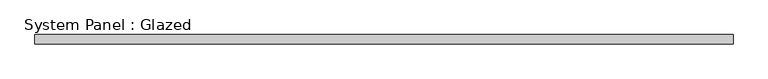
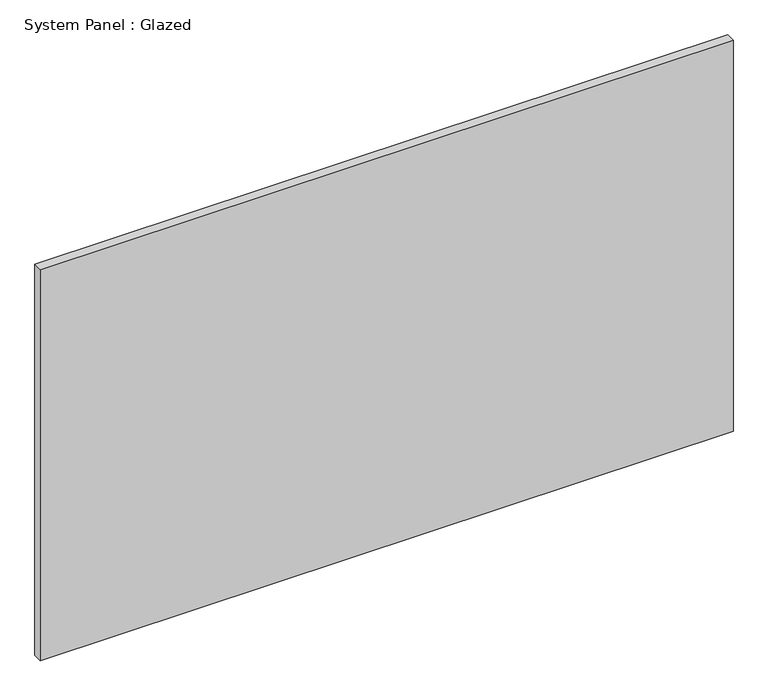
"""IFC4 building model written with IfcOpenShell, lengths in millimetres: plate geometry, System Panel : Glazed."""

from ifc_helpers import new_model, si_unit, origin, origin_with_axes, place, context, project, spatial, polyline, outline, extrude, source, transform, mapped, element, save


def system_panel_glazed_a2373be0(model_context):
    return source(origin(), model_context, "Body", "SweptSolid", [
        extrude(outline(polyline([(968.375, -44.45), (-968.375, -44.45), (-968.375, -19.05), (968.375, -19.05), (968.375, -44.45)])), origin_with_axes(), (0.0, 0.0, 1.0), 1155.7),
    ])


if __name__ == "__main__":
    model = new_model("IFC4")
    model_context = context("Model", 3, world=origin())
    ifc_project = project(units=[si_unit("LENGTHUNIT", "METRE", prefix="MILLI")], contexts=[model_context])
    site = spatial("IfcSite", under=ifc_project)
    building = spatial("IfcBuilding", under=site)
    placement = place(None, origin())
    system_panel_glazed_shape = system_panel_glazed_a2373be0(model_context)
    element("IfcPlate", 1, ObjectType="System Panel : Glazed", at=placement, inside=building, context=model_context, shape_type="MappedRepresentation", body=[
        mapped(system_panel_glazed_shape, transform((0.0, 0.0, 0.0), x_axis=(1.0, 0.0, 0.0), y_axis=(0.0, 1.0, 0.0), z_axis=(0.0, 0.0, 1.0))),
    ])
    save(model, "model.ifc")

# Revit data of these elements
# Element 1 (IfcPlate, "System Panel : Glazed")
#   Materials on its faces: "Glass"
# Materials
#   "Glass": class "Glass", colour RGB 0 128 192, transparency 0.75
